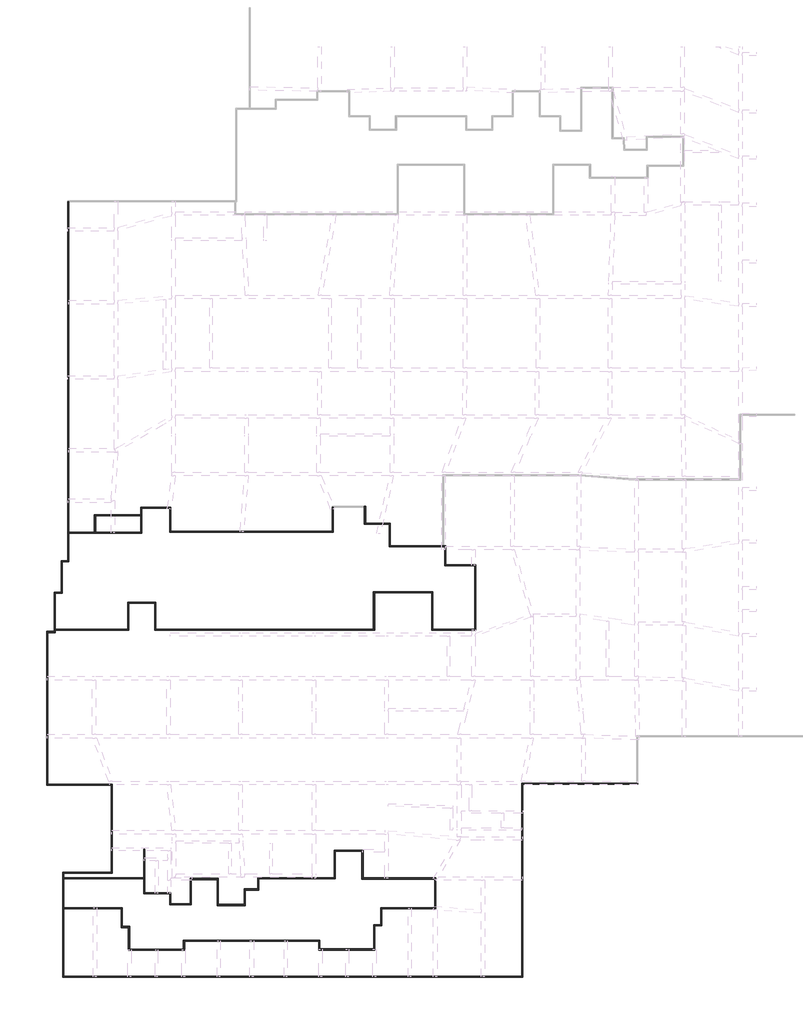
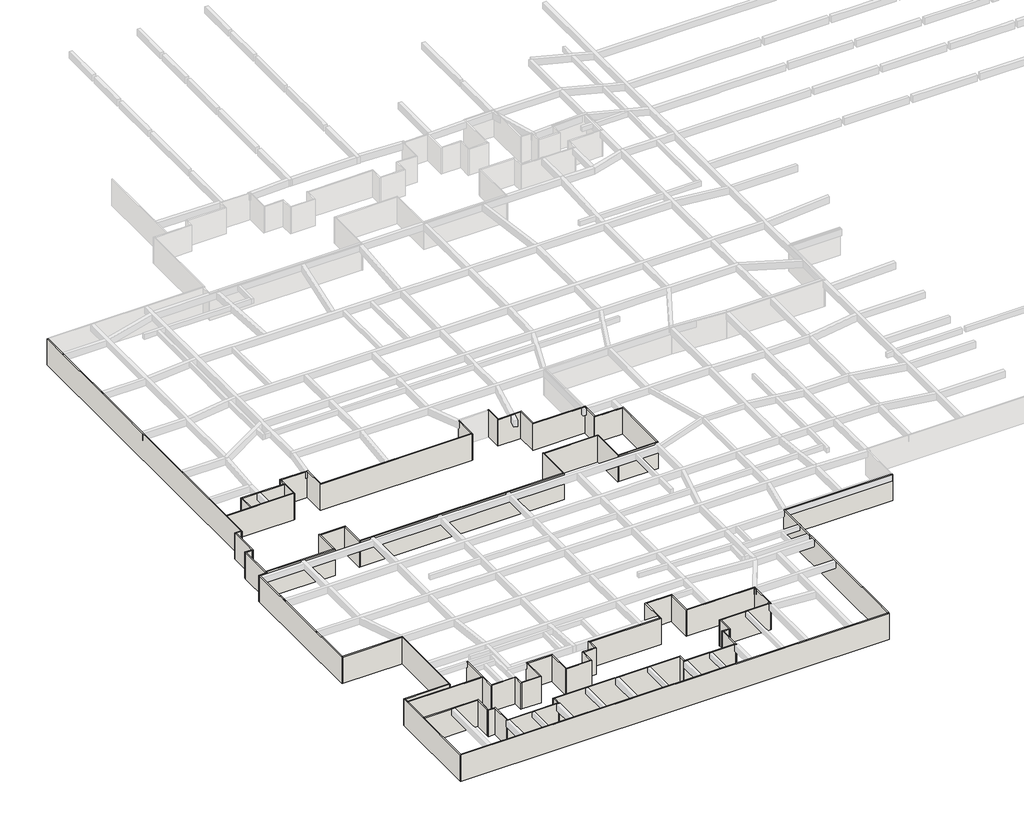
# One storey, part 1 of 16: 69 walls.
"""IFC4 building model written with IfcOpenShell, lengths in millimetres."""

from ifc_helpers import new_model, si_unit, origin, origin_with_axes, place, context, project, spatial, polyline, outline, extrude, faceted_brep, element, save

model = new_model("IFC4")

# Units and contexts
model_context = context("Model", 3, world=origin())
ifc_project = project(units=[si_unit("LENGTHUNIT", "METRE", prefix="MILLI")], contexts=[model_context])

# Site, building, storey
site = spatial("IfcSite", under=ifc_project)
building = spatial("IfcBuilding", under=site)
storey = spatial("IfcBuildingStorey", under=building, Name="户型图", Elevation=0.0)

# Walls
placement = place(None, origin())
element("IfcWall", 1, ObjectType="所有墙体", at=placement, inside=storey, context=model_context, shape_type="Brep", body=[
    faceted_brep([(66562.5546537, 146202.3185248, 0.0), (66562.5546537, 106222.3185248, 0.0), (66562.5546537, 106102.3185248, 0.0), (66562.5546537, 106102.3185248, 3300.0), (66562.5546537, 106222.3185248, 3300.0), (66562.5546537, 146202.3185248, 3300.0), (66682.5546537, 146202.3185248, 0.0), (66682.5546537, 146202.3185248, 3300.0), (66682.5546537, 109414.5259701, 3300.0), (66682.5546537, 109294.5259701, 3300.0), (66682.5546537, 106102.3185248, 3300.0), (66682.5546537, 106102.3185248, 0.0), (66682.5546537, 109294.5259701, 0.0), (66682.5546537, 109414.5259701, 0.0)], [[[0, 1, 2, 3, 4, 5]], [[6, 7, 8, 9, 10, 11, 12, 13]], [[2, 1, 0, 6, 13, 12, 11]], [[5, 4, 3, 10, 9, 8, 7]], [[0, 5, 7, 6]], [[3, 2, 11, 10]]]),
])
element("IfcWall", 2, ObjectType="所有墙体", at=placement, inside=storey, context=model_context, shape_type="Brep", body=[
    faceted_brep([(66562.5546537, 106222.3185248, 0.0), (65862.5546537, 106222.3185248, 0.0), (65862.5546537, 106222.3185248, 3300.0), (66562.5546537, 106222.3185248, 3300.0), (66562.5546537, 106102.3185248, 0.0), (66562.5546537, 106102.3185248, 3300.0), (65982.5546537, 106102.3185248, 3300.0), (65862.5546537, 106102.3185248, 3300.0), (65862.5546537, 106102.3185248, 0.0), (65982.5546537, 106102.3185248, 0.0)], [[[0, 1, 2, 3]], [[4, 5, 6, 7, 8, 9]], [[1, 0, 4, 9, 8]], [[3, 2, 7, 6, 5]], [[0, 3, 5, 4]], [[2, 1, 8, 7]]]),
])
element("IfcWall", 3, ObjectType="所有墙体", at=placement, inside=storey, context=model_context, shape_type="Brep", body=[
    faceted_brep([(65862.5546537, 106102.3185248, 0.0), (65862.5546537, 102722.3185248, 0.0), (65862.5546537, 102602.3185248, 0.0), (65862.5546537, 102602.3185248, 3300.0), (65862.5546537, 102722.3185248, 3300.0), (65862.5546537, 106102.3185248, 3300.0), (65982.5546537, 106102.3185248, 0.0), (65982.5546537, 106102.3185248, 3300.0), (65982.5546537, 102602.3185248, 3300.0), (65982.5546537, 102602.3185248, 0.0)], [[[0, 1, 2, 3, 4, 5]], [[6, 7, 8, 9]], [[2, 1, 0, 6, 9]], [[5, 4, 3, 8, 7]], [[0, 5, 7, 6]], [[3, 2, 9, 8]]]),
])
element("IfcWall", 4, ObjectType="所有墙体", at=placement, inside=storey, context=model_context, shape_type="Brep", body=[
    faceted_brep([(65862.5546537, 102722.3185248, 0.0), (65062.3671537, 102722.3185248, 0.0), (65062.3671537, 102722.3185248, 3300.0), (65862.5546537, 102722.3185248, 3300.0), (65862.5546537, 102602.3185248, 0.0), (65862.5546537, 102602.3185248, 3300.0), (65182.3671537, 102602.3185248, 3300.0), (65062.3671537, 102602.3185248, 3300.0), (65062.3671537, 102602.3185248, 0.0), (65182.3671537, 102602.3185248, 0.0)], [[[0, 1, 2, 3]], [[4, 5, 6, 7, 8, 9]], [[1, 0, 4, 9, 8]], [[3, 2, 7, 6, 5]], [[0, 3, 5, 4]], [[2, 1, 8, 7]]]),
])
element("IfcWall", 5, ObjectType="所有墙体", at=placement, inside=storey, context=model_context, shape_type="Brep", body=[
    faceted_brep([(65062.3671537, 102602.3185248, 0.0), (65062.3671537, 98364.6119076, 0.0), (65062.3671537, 98244.6119076, 0.0), (65062.3671537, 98244.6119076, 3300.0), (65062.3671537, 98364.6119076, 3300.0), (65062.3671537, 102602.3185248, 3300.0), (65182.3671537, 102602.3185248, 0.0), (65182.3671537, 102602.3185248, 3300.0), (65182.3671537, 98614.6119076, 3300.0), (65182.3671537, 98494.6119076, 3300.0), (65182.3671537, 98244.6119076, 3300.0), (65182.3671537, 98244.6119076, 0.0), (65182.3671537, 98494.6119076, 0.0), (65182.3671537, 98614.6119076, 0.0)], [[[0, 1, 2, 3, 4, 5]], [[6, 7, 8, 9, 10, 11, 12, 13]], [[2, 1, 0, 6, 13, 12, 11]], [[5, 4, 3, 10, 9, 8, 7]], [[0, 5, 7, 6]], [[3, 2, 11, 10]]]),
])
element("IfcWall", 6, ObjectType="所有墙体", at=placement, inside=storey, context=model_context, shape_type="Brep", body=[
    faceted_brep([(65062.3671537, 98364.6119076, 0.0), (64221.0654488, 98364.6119076, 0.0), (64221.0654488, 98364.6119076, 3300.0), (65062.3671537, 98364.6119076, 3300.0), (65062.3671537, 98244.6119076, 0.0), (65062.3671537, 98244.6119076, 3300.0), (64341.0654488, 98244.6119076, 3300.0), (64221.0654488, 98244.6119076, 3300.0), (64221.0654488, 98244.6119076, 0.0), (64341.0654488, 98244.6119076, 0.0)], [[[0, 1, 2, 3]], [[4, 5, 6, 7, 8, 9]], [[1, 0, 4, 9, 8]], [[3, 2, 7, 6, 5]], [[0, 3, 5, 4]], [[2, 1, 8, 7]]]),
])
element("IfcWall", 7, ObjectType="所有墙体", at=placement, inside=storey, context=model_context, shape_type="Brep", body=[
    faceted_brep([(64221.0654488, 98244.6119076, 0.0), (64221.0654488, 81244.6119076, 0.0), (64221.0654488, 81244.6119076, 3300.0), (64221.0654488, 98244.6119076, 3300.0), (64341.0654488, 98244.6119076, 0.0), (64341.0654488, 98244.6119076, 3300.0), (64341.0654488, 81364.6119076, 3300.0), (64341.0654488, 81244.6119076, 3300.0), (64341.0654488, 81244.6119076, 0.0), (64341.0654488, 81364.6119076, 0.0)], [[[0, 1, 2, 3]], [[4, 5, 6, 7, 8, 9]], [[1, 0, 4, 9, 8]], [[3, 2, 7, 6, 5]], [[0, 3, 5, 4]], [[2, 1, 8, 7]]]),
])
element("IfcWall", 8, ObjectType="所有墙体", at=placement, inside=storey, context=model_context, shape_type="Brep", body=[
    faceted_brep([(64341.0654488, 81244.6119076, 0.0), (71421.0654488, 81244.6119076, 0.0), (71541.0654488, 81244.6119076, 0.0), (71541.0654488, 81244.6119076, 3300.0), (71421.0654488, 81244.6119076, 3300.0), (64341.0654488, 81244.6119076, 3300.0), (64341.0654488, 81364.6119076, 0.0), (64341.0654488, 81364.6119076, 3300.0), (71541.0654488, 81364.6119076, 3300.0), (71541.0654488, 81364.6119076, 0.0)], [[[0, 1, 2, 3, 4, 5]], [[6, 7, 8, 9]], [[2, 1, 0, 6, 9]], [[5, 4, 3, 8, 7]], [[0, 5, 7, 6]], [[3, 2, 9, 8]]]),
])
element("IfcWall", 9, ObjectType="所有墙体", at=placement, inside=storey, context=model_context, shape_type="Brep", body=[
    faceted_brep([(71421.0654488, 81244.6119076, 0.0), (71421.0654488, 71564.6119076, 0.0), (71421.0654488, 71444.6119076, 0.0), (71421.0654488, 71444.6119076, 3300.0), (71421.0654488, 71564.6119076, 3300.0), (71421.0654488, 81244.6119076, 3300.0), (71541.0654488, 81244.6119076, 0.0), (71541.0654488, 81244.6119076, 3300.0), (71541.0654488, 71444.6119076, 3300.0), (71541.0654488, 71444.6119076, 0.0)], [[[0, 1, 2, 3, 4, 5]], [[6, 7, 8, 9]], [[2, 1, 0, 6, 9]], [[5, 4, 3, 8, 7]], [[0, 5, 7, 6]], [[3, 2, 9, 8]]]),
])
element("IfcWall", 10, ObjectType="所有墙体", at=placement, inside=storey, context=model_context, shape_type="Brep", body=[
    faceted_brep([(71421.0654488, 71564.6119076, 0.0), (66021.0654488, 71564.6119076, 0.0), (66021.0654488, 71564.6119076, 3300.0), (71421.0654488, 71564.6119076, 3300.0), (71421.0654488, 71444.6119076, 0.0), (71421.0654488, 71444.6119076, 3300.0), (66141.0654488, 71444.6119076, 3300.0), (66021.0654488, 71444.6119076, 3300.0), (66021.0654488, 71444.6119076, 0.0), (66141.0654488, 71444.6119076, 0.0)], [[[0, 1, 2, 3]], [[4, 5, 6, 7, 8, 9]], [[1, 0, 4, 9, 8]], [[3, 2, 7, 6, 5]], [[0, 3, 5, 4]], [[2, 1, 8, 7]]]),
])
element("IfcWall", 11, ObjectType="所有墙体", at=placement, inside=storey, context=model_context, shape_type="Brep", body=[
    faceted_brep([(66021.0654488, 71444.6119076, 0.0), (66021.0654488, 59844.6119076, 0.0), (66021.0654488, 59844.6119076, 3300.0), (66021.0654488, 71444.6119076, 3300.0), (66141.0654488, 71444.6119076, 0.0), (66141.0654488, 71444.6119076, 3300.0), (66141.0654488, 70967.5572201, 3300.0), (66141.0654488, 70847.5572201, 3300.0), (66141.0654488, 67617.5941469, 3300.0), (66141.0654488, 67497.5941469, 3300.0), (66141.0654488, 59964.6119076, 3300.0), (66141.0654488, 59844.6119076, 3300.0), (66141.0654488, 59844.6119076, 0.0), (66141.0654488, 59964.6119076, 0.0), (66141.0654488, 67497.5941469, 0.0), (66141.0654488, 67617.5941469, 0.0), (66141.0654488, 70847.5572201, 0.0), (66141.0654488, 70967.5572201, 0.0)], [[[0, 1, 2, 3]], [[4, 5, 6, 7, 8, 9, 10, 11, 12, 13, 14, 15, 16, 17]], [[1, 0, 4, 17, 16, 15, 14, 13, 12]], [[3, 2, 11, 10, 9, 8, 7, 6, 5]], [[0, 3, 5, 4]], [[2, 1, 12, 11]]]),
])
element("IfcWall", 12, ObjectType="所有墙体", at=placement, inside=storey, context=model_context, shape_type="Brep", body=[
    faceted_brep([(66141.0654488, 59844.6119076, 0.0), (117241.0654488, 59844.6119076, 0.0), (117241.0654488, 59844.6119076, 3300.0), (66141.0654488, 59844.6119076, 3300.0), (66141.0654488, 59964.6119076, 0.0), (66141.0654488, 59964.6119076, 3300.0), (117121.0654488, 59964.6119076, 3300.0), (117241.0654488, 59964.6119076, 3300.0), (117241.0654488, 59964.6119076, 0.0), (117121.0654488, 59964.6119076, 0.0)], [[[0, 1, 2, 3]], [[4, 5, 6, 7, 8, 9]], [[1, 0, 4, 9, 8]], [[3, 2, 7, 6, 5]], [[0, 3, 5, 4]], [[2, 1, 8, 7]]]),
])
element("IfcWall", 13, ObjectType="所有墙体", at=placement, inside=storey, context=model_context, shape_type="Brep", body=[
    faceted_brep([(117241.0654488, 59964.6119076, 0.0), (117241.0654488, 81344.6119076, 0.0), (117241.0654488, 81464.6119076, 0.0), (117241.0654488, 81464.6119076, 3300.0), (117241.0654488, 81344.6119076, 3300.0), (117241.0654488, 59964.6119076, 3300.0), (117121.0654488, 59964.6119076, 0.0), (117121.0654488, 59964.6119076, 3300.0), (117121.0654488, 81464.6119076, 3300.0), (117121.0654488, 81464.6119076, 0.0)], [[[0, 1, 2, 3, 4, 5]], [[6, 7, 8, 9]], [[2, 1, 0, 6, 9]], [[5, 4, 3, 8, 7]], [[0, 5, 7, 6]], [[3, 2, 9, 8]]]),
])
element("IfcWall", 14, ObjectType="所有墙体", at=placement, inside=storey, context=model_context, shape_type="Brep", body=[
    faceted_brep([(117241.0654488, 81344.6119076, 0.0), (130041.0654488, 81344.6119076, 0.0), (130041.0654488, 81344.6119076, 3300.0), (117241.0654488, 81344.6119076, 3300.0), (117241.0654488, 81464.6119076, 0.0), (117241.0654488, 81464.6119076, 3300.0), (129921.0654488, 81464.6119076, 3300.0), (130041.0654488, 81464.6119076, 3300.0), (130041.0654488, 81464.6119076, 0.0), (129921.0654488, 81464.6119076, 0.0)], [[[0, 1, 2, 3]], [[4, 5, 6, 7, 8, 9]], [[1, 0, 4, 9, 8]], [[3, 2, 7, 6, 5]], [[0, 3, 5, 4]], [[2, 1, 8, 7]]]),
])
element("IfcWall", 15, ObjectType="所有墙体", at=placement, inside=storey, context=model_context, shape_type="Brep", body=[
    faceted_brep([(65182.3671537, 98494.6119076, 0.0), (73382.3671537, 98494.6119076, 0.0), (73382.3671537, 98494.6119076, 3300.0), (65182.3671537, 98494.6119076, 3300.0), (65182.3671537, 98614.6119076, 0.0), (65182.3671537, 98614.6119076, 3300.0), (73262.3671537, 98614.6119076, 3300.0), (73382.3671537, 98614.6119076, 3300.0), (73382.3671537, 98614.6119076, 0.0), (73262.3671537, 98614.6119076, 0.0)], [[[0, 1, 2, 3]], [[4, 5, 6, 7, 8, 9]], [[1, 0, 4, 9, 8]], [[3, 2, 7, 6, 5]], [[0, 3, 5, 4]], [[2, 1, 8, 7]]]),
])
element("IfcWall", 16, ObjectType="所有墙体", at=placement, inside=storey, context=model_context, shape_type="Brep", body=[
    faceted_brep([(73382.3671537, 98614.6119076, 0.0), (73382.3671537, 101494.6119076, 0.0), (73382.3671537, 101614.6119076, 0.0), (73382.3671537, 101614.6119076, 3300.0), (73382.3671537, 101494.6119076, 3300.0), (73382.3671537, 98614.6119076, 3300.0), (73262.3671537, 98614.6119076, 0.0), (73262.3671537, 98614.6119076, 3300.0), (73262.3671537, 101614.6119076, 3300.0), (73262.3671537, 101614.6119076, 0.0)], [[[0, 1, 2, 3, 4, 5]], [[6, 7, 8, 9]], [[2, 1, 0, 6, 9]], [[5, 4, 3, 8, 7]], [[0, 5, 7, 6]], [[3, 2, 9, 8]]]),
])
element("IfcWall", 17, ObjectType="所有墙体", at=placement, inside=storey, context=model_context, shape_type="Brep", body=[
    faceted_brep([(73382.3671537, 101494.6119076, 0.0), (76262.3671537, 101494.6119076, 0.0), (76382.3671537, 101494.6119076, 0.0), (76382.3671537, 101494.6119076, 3300.0), (76262.3671537, 101494.6119076, 3300.0), (73382.3671537, 101494.6119076, 3300.0), (73382.3671537, 101614.6119076, 0.0), (73382.3671537, 101614.6119076, 3300.0), (76382.3671537, 101614.6119076, 3300.0), (76382.3671537, 101614.6119076, 0.0)], [[[0, 1, 2, 3, 4, 5]], [[6, 7, 8, 9]], [[2, 1, 0, 6, 9]], [[5, 4, 3, 8, 7]], [[0, 5, 7, 6]], [[3, 2, 9, 8]]]),
])
element("IfcWall", 18, ObjectType="所有墙体", at=placement, inside=storey, context=model_context, shape_type="Brep", body=[
    faceted_brep([(76262.3671537, 101494.6119076, 0.0), (76262.3671537, 98494.6092221, 0.0), (76262.3671537, 98494.6092221, 3300.0), (76262.3671537, 101494.6119076, 3300.0), (76382.3671537, 101494.6119076, 0.0), (76382.3671537, 101494.6119076, 3300.0), (76382.3671537, 98614.6092221, 3300.0), (76382.3671537, 98494.6092221, 3300.0), (76382.3671537, 98494.6092221, 0.0), (76382.3671537, 98614.6092221, 0.0)], [[[0, 1, 2, 3]], [[4, 5, 6, 7, 8, 9]], [[1, 0, 4, 9, 8]], [[3, 2, 7, 6, 5]], [[0, 3, 5, 4]], [[2, 1, 8, 7]]]),
])
element("IfcWall", 19, ObjectType="所有墙体", at=placement, inside=storey, context=model_context, shape_type="Brep", body=[
    faceted_brep([(76382.3671537, 98494.6092221, 0.0), (100732.3549466, 98494.6092221, 0.0), (100732.3549466, 98494.6092221, 3300.0), (76382.3671537, 98494.6092221, 3300.0), (76382.3671537, 98614.6092221, 0.0), (76382.3671537, 98614.6092221, 3300.0), (100612.3549466, 98614.6092221, 3300.0), (100732.3549466, 98614.6092221, 3300.0), (100732.3549466, 98614.6092221, 0.0), (100612.3549466, 98614.6092221, 0.0)], [[[0, 1, 2, 3]], [[4, 5, 6, 7, 8, 9]], [[1, 0, 4, 9, 8]], [[3, 2, 7, 6, 5]], [[0, 3, 5, 4]], [[2, 1, 8, 7]]]),
])
element("IfcWall", 20, ObjectType="所有墙体", at=placement, inside=storey, context=model_context, shape_type="Brep", body=[
    faceted_brep([(100732.3549466, 98614.6092221, 0.0), (100732.3549466, 102644.6089779, 0.0), (100732.3549466, 102764.6089779, 0.0), (100732.3549466, 102764.6089779, 3300.0), (100732.3549466, 102644.6089779, 3300.0), (100732.3549466, 98614.6092221, 3300.0), (100612.3549466, 98614.6092221, 0.0), (100612.3549466, 98614.6092221, 3300.0), (100612.3549466, 102764.6089779, 3300.0), (100612.3549466, 102764.6089779, 0.0)], [[[0, 1, 2, 3, 4, 5]], [[6, 7, 8, 9]], [[2, 1, 0, 6, 9]], [[5, 4, 3, 8, 7]], [[0, 5, 7, 6]], [[3, 2, 9, 8]]]),
])
element("IfcWall", 21, ObjectType="所有墙体", at=placement, inside=storey, context=model_context, shape_type="Brep", body=[
    faceted_brep([(100732.3549466, 102644.6089779, 0.0), (107112.3549466, 102644.6089779, 0.0), (107232.3549466, 102644.6089779, 0.0), (107232.3549466, 102644.6089779, 3300.0), (107112.3549466, 102644.6089779, 3300.0), (100732.3549466, 102644.6089779, 3300.0), (100732.3549466, 102764.6089779, 0.0), (100732.3549466, 102764.6089779, 3300.0), (107232.3549466, 102764.6089779, 3300.0), (107232.3549466, 102764.6089779, 0.0)], [[[0, 1, 2, 3, 4, 5]], [[6, 7, 8, 9]], [[2, 1, 0, 6, 9]], [[5, 4, 3, 8, 7]], [[0, 5, 7, 6]], [[3, 2, 9, 8]]]),
])
element("IfcWall", 22, ObjectType="所有墙体", at=placement, inside=storey, context=model_context, shape_type="Brep", body=[
    faceted_brep([(107112.3549466, 102644.6089779, 0.0), (107112.3549466, 98494.6092221, 0.0), (107112.3549466, 98494.6092221, 3300.0), (107112.3549466, 102644.6089779, 3300.0), (107232.3549466, 102644.6089779, 0.0), (107232.3549466, 102644.6089779, 3300.0), (107232.3549466, 98614.6092221, 3300.0), (107232.3549466, 98494.6092221, 3300.0), (107232.3549466, 98494.6092221, 0.0), (107232.3549466, 98614.6092221, 0.0)], [[[0, 1, 2, 3]], [[4, 5, 6, 7, 8, 9]], [[1, 0, 4, 9, 8]], [[3, 2, 7, 6, 5]], [[0, 3, 5, 4]], [[2, 1, 8, 7]]]),
])
element("IfcWall", 23, ObjectType="所有墙体", at=placement, inside=storey, context=model_context, shape_type="Brep", body=[
    faceted_brep([(107232.3549466, 98494.6092221, 0.0), (111982.3392399, 98494.6092221, 0.0), (111982.3392399, 98494.6092221, 3300.0), (107232.3549466, 98494.6092221, 3300.0), (107232.3549466, 98614.6092221, 0.0), (107232.3549466, 98614.6092221, 3300.0), (111862.3392399, 98614.6092221, 3300.0), (111982.3392399, 98614.6092221, 3300.0), (111982.3392399, 98614.6092221, 0.0), (111862.3392399, 98614.6092221, 0.0)], [[[0, 1, 2, 3]], [[4, 5, 6, 7, 8, 9]], [[1, 0, 4, 9, 8]], [[3, 2, 7, 6, 5]], [[0, 3, 5, 4]], [[2, 1, 8, 7]]]),
])
element("IfcWall", 24, ObjectType="所有墙体", at=placement, inside=storey, context=model_context, shape_type="Brep", body=[
    faceted_brep([(111982.3392399, 98614.6092221, 0.0), (111982.3392399, 105814.6092221, 0.0), (111982.3392399, 105814.6092221, 3300.0), (111982.3392399, 98614.6092221, 3300.0), (111862.3392399, 98614.6092221, 0.0), (111862.3392399, 98614.6092221, 3300.0), (111862.3392399, 105694.6092221, 3300.0), (111862.3392399, 105814.6092221, 3300.0), (111862.3392399, 105814.6092221, 0.0), (111862.3392399, 105694.6092221, 0.0)], [[[0, 1, 2, 3]], [[4, 5, 6, 7, 8, 9]], [[1, 0, 4, 9, 8]], [[3, 2, 7, 6, 5]], [[0, 3, 5, 4]], [[2, 1, 8, 7]]]),
])
element("IfcWall", 25, ObjectType="所有墙体", at=placement, inside=storey, context=model_context, shape_type="Brep", body=[
    faceted_brep([(111862.3392399, 105814.6092221, 0.0), (108682.3515287, 105814.6092221, 0.0), (108562.3515287, 105814.6092221, 0.0), (108562.3515287, 105814.6092221, 3300.0), (108682.3515287, 105814.6092221, 3300.0), (111862.3392399, 105814.6092221, 3300.0), (111862.3392399, 105694.6092221, 0.0), (111862.3392399, 105694.6092221, 3300.0), (108562.3515287, 105694.6092221, 3300.0), (108562.3515287, 105694.6092221, 0.0)], [[[0, 1, 2, 3, 4, 5]], [[6, 7, 8, 9]], [[2, 1, 0, 6, 9]], [[5, 4, 3, 8, 7]], [[0, 5, 7, 6]], [[3, 2, 9, 8]]]),
])
element("IfcWall", 26, ObjectType="所有墙体", at=placement, inside=storey, context=model_context, shape_type="Brep", body=[
    faceted_brep([(108682.3515287, 105814.6092221, 0.0), (108682.3515287, 107920.5715249, 0.0), (108682.3515287, 107920.5715249, 3300.0), (108682.3515287, 105814.6092221, 3300.0), (108562.3515287, 105814.6092221, 0.0), (108562.3515287, 105814.6092221, 3300.0), (108562.3515287, 107800.5715249, 3300.0), (108562.3515287, 107920.5715249, 3300.0), (108562.3515287, 107920.5715249, 0.0), (108562.3515287, 107800.5715249, 0.0)], [[[0, 1, 2, 3]], [[4, 5, 6, 7, 8, 9]], [[1, 0, 4, 9, 8]], [[3, 2, 7, 6, 5]], [[0, 3, 5, 4]], [[2, 1, 8, 7]]]),
])
element("IfcWall", 27, ObjectType="所有墙体", at=placement, inside=storey, context=model_context, shape_type="Brep", body=[
    faceted_brep([(108562.3515287, 107920.5715249, 0.0), (108444.4540331, 107920.5715249, 0.0), (108324.4540331, 107920.5715249, 0.0), (102482.3515287, 107920.5715249, 0.0), (102362.3515287, 107920.5715249, 0.0), (102362.3515287, 107920.5715249, 3300.0), (102482.3515287, 107920.5715249, 3300.0), (108324.4540331, 107920.5715249, 3300.0), (108444.4540331, 107920.5715249, 3300.0), (108562.3515287, 107920.5715249, 3300.0), (108562.3515287, 107800.5715249, 0.0), (108562.3515287, 107800.5715249, 3300.0), (102362.3515287, 107800.5715249, 3300.0), (102362.3515287, 107800.5715249, 0.0)], [[[0, 1, 2, 3, 4, 5, 6, 7, 8, 9]], [[10, 11, 12, 13]], [[4, 3, 2, 1, 0, 10, 13]], [[9, 8, 7, 6, 5, 12, 11]], [[0, 9, 11, 10]], [[5, 4, 13, 12]]]),
])
element("IfcWall", 28, ObjectType="所有墙体", at=placement, inside=storey, context=model_context, shape_type="Brep", body=[
    faceted_brep([(102482.3515287, 107920.5715249, 0.0), (102482.3515287, 110420.5715249, 0.0), (102482.3515287, 110420.5715249, 3300.0), (102482.3515287, 107920.5715249, 3300.0), (102362.3515287, 107920.5715249, 0.0), (102362.3515287, 107920.5715249, 3300.0), (102362.3515287, 110300.5715249, 3300.0), (102362.3515287, 110420.5715249, 3300.0), (102362.3515287, 110420.5715249, 0.0), (102362.3515287, 110300.5715249, 0.0)], [[[0, 1, 2, 3]], [[4, 5, 6, 7, 8, 9]], [[1, 0, 4, 9, 8]], [[3, 2, 7, 6, 5]], [[0, 3, 5, 4]], [[2, 1, 8, 7]]]),
])
element("IfcWall", 29, ObjectType="所有墙体", at=placement, inside=storey, context=model_context, shape_type="Brep", body=[
    faceted_brep([(102362.3515287, 110420.5715249, 0.0), (99732.3510404, 110420.5715249, 0.0), (99612.3510404, 110420.5715249, 0.0), (99612.3510404, 110420.5715249, 3300.0), (99732.3510404, 110420.5715249, 3300.0), (102362.3515287, 110420.5715249, 3300.0), (102362.3515287, 110300.5715249, 0.0), (102362.3515287, 110300.5715249, 3300.0), (99612.3510404, 110300.5715249, 3300.0), (99612.3510404, 110300.5715249, 0.0)], [[[0, 1, 2, 3, 4, 5]], [[6, 7, 8, 9]], [[2, 1, 0, 6, 9]], [[5, 4, 3, 8, 7]], [[0, 5, 7, 6]], [[3, 2, 9, 8]]]),
])
element("IfcWall", 30, ObjectType="所有墙体", at=placement, inside=storey, context=model_context, shape_type="Brep", body=[
    faceted_brep([(99732.3510404, 110420.5715249, 0.0), (99732.3510404, 112314.5259701, 0.0), (99732.3510404, 112314.5259701, 3300.0), (99732.3510404, 110420.5715249, 3300.0), (99612.3510404, 110420.5715249, 0.0), (99612.3510404, 110420.5715249, 3300.0), (99612.3510404, 112194.5259701, 3300.0), (99612.3510404, 112314.5259701, 3300.0), (99612.3510404, 112314.5259701, 0.0), (99612.3510404, 112194.5259701, 0.0)], [[[0, 1, 2, 3]], [[4, 5, 6, 7, 8, 9]], [[1, 0, 4, 9, 8]], [[3, 2, 7, 6, 5]], [[0, 3, 5, 4]], [[2, 1, 8, 7]]]),
])
element("IfcWall", 31, ObjectType="所有墙体", at=placement, inside=storey, context=model_context, shape_type="Brep", body=[
    faceted_brep([(96012.3510404, 112194.5259701, 0.0), (96012.3510404, 109514.5259701, 0.0), (96012.3510404, 109394.5259701, 0.0), (96012.3510404, 109394.5259701, 3300.0), (96012.3510404, 109514.5259701, 3300.0), (96012.3510404, 112194.5259701, 3300.0), (96132.3510404, 112194.5259701, 0.0), (96132.3510404, 112194.5259701, 3300.0), (96132.3510404, 109394.5259701, 3300.0), (96132.3510404, 109394.5259701, 0.0)], [[[0, 1, 2, 3, 4, 5]], [[6, 7, 8, 9]], [[2, 1, 0, 6, 9]], [[5, 4, 3, 8, 7]], [[0, 5, 7, 6]], [[3, 2, 9, 8]]]),
])
element("IfcWall", 32, ObjectType="所有墙体", at=placement, inside=storey, context=model_context, shape_type="Brep", body=[
    faceted_brep([(96012.3510404, 109514.5259701, 0.0), (78032.3510404, 109514.5259701, 0.0), (77912.3510404, 109514.5259701, 0.0), (77912.3510404, 109514.5259701, 3300.0), (78032.3510404, 109514.5259701, 3300.0), (96012.3510404, 109514.5259701, 3300.0), (96012.3510404, 109394.5259701, 0.0), (96012.3510404, 109394.5259701, 3300.0), (77912.3510404, 109394.5259701, 3300.0), (77912.3510404, 109394.5259701, 0.0)], [[[0, 1, 2, 3, 4, 5]], [[6, 7, 8, 9]], [[2, 1, 0, 6, 9]], [[5, 4, 3, 8, 7]], [[0, 5, 7, 6]], [[3, 2, 9, 8]]]),
])
element("IfcWall", 33, ObjectType="所有墙体", at=placement, inside=storey, context=model_context, shape_type="Brep", body=[
    faceted_brep([(78032.3510404, 109514.5259701, 0.0), (78032.3510404, 112214.5259701, 0.0), (78032.3510404, 112214.5259701, 3300.0), (78032.3510404, 109514.5259701, 3300.0), (77912.3510404, 109514.5259701, 0.0), (77912.3510404, 109514.5259701, 3300.0), (77912.3510404, 112094.5259701, 3300.0), (77912.3510404, 112214.5259701, 3300.0), (77912.3510404, 112214.5259701, 0.0), (77912.3510404, 112094.5259701, 0.0)], [[[0, 1, 2, 3]], [[4, 5, 6, 7, 8, 9]], [[1, 0, 4, 9, 8]], [[3, 2, 7, 6, 5]], [[0, 3, 5, 4]], [[2, 1, 8, 7]]]),
])
element("IfcWall", 34, ObjectType="所有墙体", at=placement, inside=storey, context=model_context, shape_type="Brep", body=[
    faceted_brep([(77912.3510404, 112214.5259701, 0.0), (74712.3510404, 112214.5259701, 0.0), (74712.3510404, 112214.5259701, 3300.0), (77912.3510404, 112214.5259701, 3300.0), (77912.3510404, 112094.5259701, 0.0), (77912.3510404, 112094.5259701, 3300.0), (74832.3510404, 112094.5259701, 3300.0), (74712.3510404, 112094.5259701, 3300.0), (74712.3510404, 112094.5259701, 0.0), (74832.3510404, 112094.5259701, 0.0)], [[[0, 1, 2, 3]], [[4, 5, 6, 7, 8, 9]], [[1, 0, 4, 9, 8]], [[3, 2, 7, 6, 5]], [[0, 3, 5, 4]], [[2, 1, 8, 7]]]),
])
element("IfcWall", 35, ObjectType="所有墙体", at=placement, inside=storey, context=model_context, shape_type="Brep", body=[
    faceted_brep([(74712.3510404, 112094.5259701, 0.0), (74712.3510404, 111354.5259701, 0.0), (74712.3510404, 111234.5259701, 0.0), (74712.3510404, 109414.5259701, 0.0), (74712.3510404, 109294.5259701, 0.0), (74712.3510404, 109294.5259701, 3300.0), (74712.3510404, 109414.5259701, 3300.0), (74712.3510404, 111234.5259701, 3300.0), (74712.3510404, 111354.5259701, 3300.0), (74712.3510404, 112094.5259701, 3300.0), (74832.3510404, 112094.5259701, 0.0), (74832.3510404, 112094.5259701, 3300.0), (74832.3510404, 109294.5259701, 3300.0), (74832.3510404, 109294.5259701, 0.0)], [[[0, 1, 2, 3, 4, 5, 6, 7, 8, 9]], [[10, 11, 12, 13]], [[4, 3, 2, 1, 0, 10, 13]], [[9, 8, 7, 6, 5, 12, 11]], [[0, 9, 11, 10]], [[5, 4, 13, 12]]]),
])
element("IfcWall", 36, ObjectType="所有墙体", at=placement, inside=storey, context=model_context, shape_type="Brep", body=[
    faceted_brep([(74712.3510404, 109414.5259701, 0.0), (69672.3510404, 109414.5259701, 0.0), (69552.3510404, 109414.5259701, 0.0), (66682.5546537, 109414.5259701, 0.0), (66682.5546537, 109414.5259701, 3300.0), (69552.3510404, 109414.5259701, 3300.0), (69672.3510404, 109414.5259701, 3300.0), (74712.3510404, 109414.5259701, 3300.0), (74712.3510404, 109294.5259701, 0.0), (74712.3510404, 109294.5259701, 3300.0), (66682.5546537, 109294.5259701, 3300.0), (66682.5546537, 109294.5259701, 0.0)], [[[0, 1, 2, 3, 4, 5, 6, 7]], [[8, 9, 10, 11]], [[3, 2, 1, 0, 8, 11]], [[7, 6, 5, 4, 10, 9]], [[0, 7, 9, 8]], [[4, 3, 11, 10]]]),
])
element("IfcWall", 37, ObjectType="所有墙体", at=placement, inside=storey, context=model_context, shape_type="Brep", body=[
    faceted_brep([(74712.3510404, 111354.5259701, 0.0), (69552.3510404, 111354.5259701, 0.0), (69552.3510404, 111354.5259701, 3300.0), (74712.3510404, 111354.5259701, 3300.0), (74712.3510404, 111234.5259701, 0.0), (74712.3510404, 111234.5259701, 3300.0), (69672.3510404, 111234.5259701, 3300.0), (69552.3510404, 111234.5259701, 3300.0), (69552.3510404, 111234.5259701, 0.0), (69672.3510404, 111234.5259701, 0.0)], [[[0, 1, 2, 3]], [[4, 5, 6, 7, 8, 9]], [[1, 0, 4, 9, 8]], [[3, 2, 7, 6, 5]], [[0, 3, 5, 4]], [[2, 1, 8, 7]]]),
])
element("IfcWall", 38, ObjectType="所有墙体", at=placement, inside=storey, context=model_context, shape_type="SweptSolid", body=[
    extrude(outline(polyline([(69552.3510404, 109414.5259701), (69552.3510404, 111234.5259701), (69672.3510404, 111234.5259701), (69672.3510404, 109414.5259701), (69552.3510404, 109414.5259701)])), origin_with_axes(), (0.0, 0.0, 1.0), 3300.0),
])
element("IfcWall", 39, ObjectType="所有墙体", at=placement, inside=storey, context=model_context, shape_type="SweptSolid", body=[
    extrude(outline(polyline([(75021.0654488, 70847.5572201), (66141.0654488, 70847.5572201), (66141.0654488, 70967.5572201), (75021.0654488, 70967.5572201), (75021.0654488, 70847.5572201)])), origin_with_axes(), (0.0, 0.0, 1.0), 3300.0),
])
element("IfcWall", 40, ObjectType="所有墙体", at=placement, inside=storey, context=model_context, shape_type="Brep", body=[
    faceted_brep([(75141.0654488, 69147.5572201, 0.0), (75141.0654488, 69267.5572201, 0.0), (75141.0654488, 74107.5572201, 0.0), (75141.0654488, 74107.5572201, 3300.0), (75141.0654488, 69267.5572201, 3300.0), (75141.0654488, 69147.5572201, 3300.0), (75021.0654488, 69147.5572201, 0.0), (75021.0654488, 69147.5572201, 3300.0), (75021.0654488, 70847.5572201, 3300.0), (75021.0654488, 70967.5572201, 3300.0), (75021.0654488, 74107.5572201, 3300.0), (75021.0654488, 74107.5572201, 0.0), (75021.0654488, 70967.5572201, 0.0), (75021.0654488, 70847.5572201, 0.0)], [[[0, 1, 2, 3, 4, 5]], [[6, 7, 8, 9, 10, 11, 12, 13]], [[2, 1, 0, 6, 13, 12, 11]], [[3, 2, 11, 10]], [[5, 4, 3, 10, 9, 8, 7]], [[0, 5, 7, 6]]]),
])
element("IfcWall", 41, ObjectType="所有墙体", at=placement, inside=storey, context=model_context, shape_type="Brep", body=[
    faceted_brep([(75141.0654488, 69147.5572201, 0.0), (77937.2421537, 69147.5572201, 0.0), (78057.2421537, 69147.5572201, 0.0), (78057.2421537, 69147.5572201, 3300.0), (77937.2421537, 69147.5572201, 3300.0), (75141.0654488, 69147.5572201, 3300.0), (75141.0654488, 69267.5572201, 0.0), (75141.0654488, 69267.5572201, 3300.0), (78057.2421537, 69267.5572201, 3300.0), (78057.2421537, 69267.5572201, 0.0)], [[[0, 1, 2, 3, 4, 5]], [[6, 7, 8, 9]], [[2, 1, 0, 6, 9]], [[5, 4, 3, 8, 7]], [[0, 5, 7, 6]], [[3, 2, 9, 8]]]),
])
element("IfcWall", 42, ObjectType="所有墙体", at=placement, inside=storey, context=model_context, shape_type="Brep", body=[
    faceted_brep([(77937.2421537, 69147.5572201, 0.0), (77937.2421537, 67947.5572201, 0.0), (77937.2421537, 67947.5572201, 3300.0), (77937.2421537, 69147.5572201, 3300.0), (78057.2421537, 69147.5572201, 0.0), (78057.2421537, 69147.5572201, 3300.0), (78057.2421537, 68067.5572201, 3300.0), (78057.2421537, 67947.5572201, 3300.0), (78057.2421537, 67947.5572201, 0.0), (78057.2421537, 68067.5572201, 0.0)], [[[0, 1, 2, 3]], [[4, 5, 6, 7, 8, 9]], [[1, 0, 4, 9, 8]], [[3, 2, 7, 6, 5]], [[0, 3, 5, 4]], [[2, 1, 8, 7]]]),
])
element("IfcWall", 43, ObjectType="所有墙体", at=placement, inside=storey, context=model_context, shape_type="Brep", body=[
    faceted_brep([(78057.2421537, 67947.5572201, 0.0), (80357.2421537, 67947.5572201, 0.0), (80357.2421537, 67947.5572201, 3300.0), (78057.2421537, 67947.5572201, 3300.0), (78057.2421537, 68067.5572201, 0.0), (78057.2421537, 68067.5572201, 3300.0), (80237.2421537, 68067.5572201, 3300.0), (80357.2421537, 68067.5572201, 3300.0), (80357.2421537, 68067.5572201, 0.0), (80237.2421537, 68067.5572201, 0.0)], [[[0, 1, 2, 3]], [[4, 5, 6, 7, 8, 9]], [[1, 0, 4, 9, 8]], [[3, 2, 7, 6, 5]], [[0, 3, 5, 4]], [[2, 1, 8, 7]]]),
])
element("IfcWall", 44, ObjectType="所有墙体", at=placement, inside=storey, context=model_context, shape_type="Brep", body=[
    faceted_brep([(80357.2421537, 68067.5572201, 0.0), (80357.2421537, 70747.5572201, 0.0), (80357.2421537, 70867.5572201, 0.0), (80357.2421537, 70867.5572201, 3300.0), (80357.2421537, 70747.5572201, 3300.0), (80357.2421537, 68067.5572201, 3300.0), (80237.2421537, 68067.5572201, 0.0), (80237.2421537, 68067.5572201, 3300.0), (80237.2421537, 70867.5572201, 3300.0), (80237.2421537, 70867.5572201, 0.0)], [[[0, 1, 2, 3, 4, 5]], [[6, 7, 8, 9]], [[2, 1, 0, 6, 9]], [[5, 4, 3, 8, 7]], [[0, 5, 7, 6]], [[3, 2, 9, 8]]]),
])
element("IfcWall", 45, ObjectType="所有墙体", at=placement, inside=storey, context=model_context, shape_type="Brep", body=[
    faceted_brep([(80357.2421537, 70747.5572201, 0.0), (83237.2421537, 70747.5572201, 0.0), (83357.2421537, 70747.5572201, 0.0), (83357.2421537, 70747.5572201, 3300.0), (83237.2421537, 70747.5572201, 3300.0), (80357.2421537, 70747.5572201, 3300.0), (80357.2421537, 70867.5572201, 0.0), (80357.2421537, 70867.5572201, 3300.0), (83357.2421537, 70867.5572201, 3300.0), (83357.2421537, 70867.5572201, 0.0)], [[[0, 1, 2, 3, 4, 5]], [[6, 7, 8, 9]], [[2, 1, 0, 6, 9]], [[5, 4, 3, 8, 7]], [[0, 5, 7, 6]], [[3, 2, 9, 8]]]),
])
element("IfcWall", 46, ObjectType="所有墙体", at=placement, inside=storey, context=model_context, shape_type="Brep", body=[
    faceted_brep([(83237.2421537, 70747.5572201, 0.0), (83237.2421537, 67847.5572201, 0.0), (83237.2421537, 67847.5572201, 3300.0), (83237.2421537, 70747.5572201, 3300.0), (83357.2421537, 70747.5572201, 0.0), (83357.2421537, 70747.5572201, 3300.0), (83357.2421537, 67967.5572201, 3300.0), (83357.2421537, 67847.5572201, 3300.0), (83357.2421537, 67847.5572201, 0.0), (83357.2421537, 67967.5572201, 0.0)], [[[0, 1, 2, 3]], [[4, 5, 6, 7, 8, 9]], [[1, 0, 4, 9, 8]], [[3, 2, 7, 6, 5]], [[0, 3, 5, 4]], [[2, 1, 8, 7]]]),
])
element("IfcWall", 47, ObjectType="所有墙体", at=placement, inside=storey, context=model_context, shape_type="Brep", body=[
    faceted_brep([(83357.2421537, 67847.5572201, 0.0), (86357.2421537, 67847.5572201, 0.0), (86357.2421537, 67847.5572201, 3300.0), (83357.2421537, 67847.5572201, 3300.0), (83357.2421537, 67967.5572201, 0.0), (83357.2421537, 67967.5572201, 3300.0), (86237.2421537, 67967.5572201, 3300.0), (86357.2421537, 67967.5572201, 3300.0), (86357.2421537, 67967.5572201, 0.0), (86237.2421537, 67967.5572201, 0.0)], [[[0, 1, 2, 3]], [[4, 5, 6, 7, 8, 9]], [[1, 0, 4, 9, 8]], [[3, 2, 7, 6, 5]], [[0, 3, 5, 4]], [[2, 1, 8, 7]]]),
])
element("IfcWall", 48, ObjectType="所有墙体", at=placement, inside=storey, context=model_context, shape_type="Brep", body=[
    faceted_brep([(86357.2421537, 67967.5572201, 0.0), (86357.2421537, 69572.5572201, 0.0), (86357.2421537, 69692.5572201, 0.0), (86357.2421537, 69692.5572201, 3300.0), (86357.2421537, 69572.5572201, 3300.0), (86357.2421537, 67967.5572201, 3300.0), (86237.2421537, 67967.5572201, 0.0), (86237.2421537, 67967.5572201, 3300.0), (86237.2421537, 69692.5572201, 3300.0), (86237.2421537, 69692.5572201, 0.0)], [[[0, 1, 2, 3, 4, 5]], [[6, 7, 8, 9]], [[2, 1, 0, 6, 9]], [[5, 4, 3, 8, 7]], [[0, 5, 7, 6]], [[3, 2, 9, 8]]]),
])
element("IfcWall", 49, ObjectType="所有墙体", at=placement, inside=storey, context=model_context, shape_type="Brep", body=[
    faceted_brep([(86357.2421537, 69572.5572201, 0.0), (87857.242764, 69572.5572201, 0.0), (87857.242764, 69572.5572201, 3300.0), (86357.2421537, 69572.5572201, 3300.0), (86357.2421537, 69692.5572201, 0.0), (86357.2421537, 69692.5572201, 3300.0), (87737.242764, 69692.5572201, 3300.0), (87857.242764, 69692.5572201, 3300.0), (87857.242764, 69692.5572201, 0.0), (87737.242764, 69692.5572201, 0.0)], [[[0, 1, 2, 3]], [[4, 5, 6, 7, 8, 9]], [[1, 0, 4, 9, 8]], [[3, 2, 7, 6, 5]], [[0, 3, 5, 4]], [[2, 1, 8, 7]]]),
])
element("IfcWall", 50, ObjectType="所有墙体", at=placement, inside=storey, context=model_context, shape_type="Brep", body=[
    faceted_brep([(87857.242764, 69692.5572201, 0.0), (87857.242764, 70847.5521192, 0.0), (87857.242764, 70967.5521192, 0.0), (87857.242764, 70967.5521192, 3300.0), (87857.242764, 70847.5521192, 3300.0), (87857.242764, 69692.5572201, 3300.0), (87737.242764, 69692.5572201, 0.0), (87737.242764, 69692.5572201, 3300.0), (87737.242764, 70967.5521192, 3300.0), (87737.242764, 70967.5521192, 0.0)], [[[0, 1, 2, 3, 4, 5]], [[6, 7, 8, 9]], [[2, 1, 0, 6, 9]], [[5, 4, 3, 8, 7]], [[0, 5, 7, 6]], [[3, 2, 9, 8]]]),
])
element("IfcWall", 51, ObjectType="所有墙体", at=placement, inside=storey, context=model_context, shape_type="Brep", body=[
    faceted_brep([(87857.242764, 70847.5521192, 0.0), (96357.242764, 70847.5521192, 0.0), (96357.242764, 70847.5521192, 3300.0), (87857.242764, 70847.5521192, 3300.0), (87857.242764, 70967.5521192, 0.0), (87857.242764, 70967.5521192, 3300.0), (96237.242764, 70967.5521192, 3300.0), (96357.242764, 70967.5521192, 3300.0), (96357.242764, 70967.5521192, 0.0), (96237.242764, 70967.5521192, 0.0)], [[[0, 1, 2, 3]], [[4, 5, 6, 7, 8, 9]], [[1, 0, 4, 9, 8]], [[3, 2, 7, 6, 5]], [[0, 3, 5, 4]], [[2, 1, 8, 7]]]),
])
element("IfcWall", 52, ObjectType="所有墙体", at=placement, inside=storey, context=model_context, shape_type="Brep", body=[
    faceted_brep([(96357.242764, 70967.5521192, 0.0), (96357.242764, 73897.5941469, 0.0), (96357.242764, 74017.5941469, 0.0), (96357.242764, 74017.5941469, 3300.0), (96357.242764, 73897.5941469, 3300.0), (96357.242764, 70967.5521192, 3300.0), (96237.242764, 70967.5521192, 0.0), (96237.242764, 70967.5521192, 3300.0), (96237.242764, 74017.5941469, 3300.0), (96237.242764, 74017.5941469, 0.0)], [[[0, 1, 2, 3, 4, 5]], [[6, 7, 8, 9]], [[2, 1, 0, 6, 9]], [[5, 4, 3, 8, 7]], [[0, 5, 7, 6]], [[3, 2, 9, 8]]]),
])
element("IfcWall", 53, ObjectType="所有墙体", at=placement, inside=storey, context=model_context, shape_type="Brep", body=[
    faceted_brep([(96357.242764, 73897.5941469, 0.0), (99335.5415162, 73897.5941469, 0.0), (99455.5415162, 73897.5941469, 0.0), (99455.5415162, 73897.5941469, 3300.0), (99335.5415162, 73897.5941469, 3300.0), (96357.242764, 73897.5941469, 3300.0), (96357.242764, 74017.5941469, 0.0), (96357.242764, 74017.5941469, 3300.0), (99455.5415162, 74017.5941469, 3300.0), (99455.5415162, 74017.5941469, 0.0)], [[[0, 1, 2, 3, 4, 5]], [[6, 7, 8, 9]], [[2, 1, 0, 6, 9]], [[5, 4, 3, 8, 7]], [[0, 5, 7, 6]], [[3, 2, 9, 8]]]),
])
element("IfcWall", 54, ObjectType="所有墙体", at=placement, inside=storey, context=model_context, shape_type="Brep", body=[
    faceted_brep([(99335.5415162, 73897.5941469, 0.0), (99335.5415162, 70797.5941469, 0.0), (99335.5415162, 70797.5941469, 3300.0), (99335.5415162, 73897.5941469, 3300.0), (99455.5415162, 73897.5941469, 0.0), (99455.5415162, 73897.5941469, 3300.0), (99455.5415162, 70917.5941469, 3300.0), (99455.5415162, 70797.5941469, 3300.0), (99455.5415162, 70797.5941469, 0.0), (99455.5415162, 70917.5941469, 0.0)], [[[0, 1, 2, 3]], [[4, 5, 6, 7, 8, 9]], [[1, 0, 4, 9, 8]], [[3, 2, 7, 6, 5]], [[0, 3, 5, 4]], [[2, 1, 8, 7]]]),
])
element("IfcWall", 55, ObjectType="所有墙体", at=placement, inside=storey, context=model_context, shape_type="Brep", body=[
    faceted_brep([(99455.5415162, 70797.5941469, 0.0), (107435.5415162, 70797.5941469, 0.0), (107555.5415162, 70797.5941469, 0.0), (107555.5415162, 70797.5941469, 3300.0), (107435.5415162, 70797.5941469, 3300.0), (99455.5415162, 70797.5941469, 3300.0), (99455.5415162, 70917.5941469, 0.0), (99455.5415162, 70917.5941469, 3300.0), (107555.5415162, 70917.5941469, 3300.0), (107555.5415162, 70917.5941469, 0.0)], [[[0, 1, 2, 3, 4, 5]], [[6, 7, 8, 9]], [[2, 1, 0, 6, 9]], [[5, 4, 3, 8, 7]], [[0, 5, 7, 6]], [[3, 2, 9, 8]]]),
])
element("IfcWall", 56, ObjectType="所有墙体", at=placement, inside=storey, context=model_context, shape_type="Brep", body=[
    faceted_brep([(107435.5415162, 70797.5941469, 0.0), (107435.5415162, 67617.5941469, 0.0), (107435.5415162, 67497.5941469, 0.0), (107435.5415162, 67497.5941469, 3300.0), (107435.5415162, 67617.5941469, 3300.0), (107435.5415162, 70797.5941469, 3300.0), (107555.5415162, 70797.5941469, 0.0), (107555.5415162, 70797.5941469, 3300.0), (107555.5415162, 67497.5941469, 3300.0), (107555.5415162, 67497.5941469, 0.0)], [[[0, 1, 2, 3, 4, 5]], [[6, 7, 8, 9]], [[2, 1, 0, 6, 9]], [[5, 4, 3, 8, 7]], [[0, 5, 7, 6]], [[3, 2, 9, 8]]]),
])
element("IfcWall", 57, ObjectType="所有墙体", at=placement, inside=storey, context=model_context, shape_type="Brep", body=[
    faceted_brep([(107435.5415162, 67617.5941469, 0.0), (101437.0218171, 67617.5941469, 0.0), (101437.0218171, 67617.5941469, 3300.0), (107435.5415162, 67617.5941469, 3300.0), (107435.5415162, 67497.5941469, 0.0), (107435.5415162, 67497.5941469, 3300.0), (101557.0218171, 67497.5941469, 3300.0), (101437.0218171, 67497.5941469, 3300.0), (101437.0218171, 67497.5941469, 0.0), (101557.0218171, 67497.5941469, 0.0)], [[[0, 1, 2, 3]], [[4, 5, 6, 7, 8, 9]], [[1, 0, 4, 9, 8]], [[3, 2, 7, 6, 5]], [[0, 3, 5, 4]], [[2, 1, 8, 7]]]),
])
element("IfcWall", 58, ObjectType="所有墙体", at=placement, inside=storey, context=model_context, shape_type="Brep", body=[
    faceted_brep([(101437.0218171, 67497.5941469, 0.0), (101437.0218171, 65717.5941469, 0.0), (101437.0218171, 65597.5941469, 0.0), (101437.0218171, 65597.5941469, 3300.0), (101437.0218171, 65717.5941469, 3300.0), (101437.0218171, 67497.5941469, 3300.0), (101557.0218171, 67497.5941469, 0.0), (101557.0218171, 67497.5941469, 3300.0), (101557.0218171, 65597.5941469, 3300.0), (101557.0218171, 65597.5941469, 0.0)], [[[0, 1, 2, 3, 4, 5]], [[6, 7, 8, 9]], [[2, 1, 0, 6, 9]], [[5, 4, 3, 8, 7]], [[0, 5, 7, 6]], [[3, 2, 9, 8]]]),
])
element("IfcWall", 59, ObjectType="所有墙体", at=placement, inside=storey, context=model_context, shape_type="Brep", body=[
    faceted_brep([(101437.0218171, 65717.5941469, 0.0), (100637.235631, 65717.5941469, 0.0), (100637.235631, 65717.5941469, 3300.0), (101437.0218171, 65717.5941469, 3300.0), (101437.0218171, 65597.5941469, 0.0), (101437.0218171, 65597.5941469, 3300.0), (100757.235631, 65597.5941469, 3300.0), (100637.235631, 65597.5941469, 3300.0), (100637.235631, 65597.5941469, 0.0), (100757.235631, 65597.5941469, 0.0)], [[[0, 1, 2, 3]], [[4, 5, 6, 7, 8, 9]], [[1, 0, 4, 9, 8]], [[3, 2, 7, 6, 5]], [[0, 3, 5, 4]], [[2, 1, 8, 7]]]),
])
element("IfcWall", 60, ObjectType="所有墙体", at=placement, inside=storey, context=model_context, shape_type="Brep", body=[
    faceted_brep([(100637.235631, 65597.5941469, 0.0), (100637.235631, 63017.5941469, 0.0), (100637.235631, 62897.5941469, 0.0), (100637.235631, 62897.5941469, 3300.0), (100637.235631, 63017.5941469, 3300.0), (100637.235631, 65597.5941469, 3300.0), (100757.235631, 65597.5941469, 0.0), (100757.235631, 65597.5941469, 3300.0), (100757.235631, 62897.5941469, 3300.0), (100757.235631, 62897.5941469, 0.0)], [[[0, 1, 2, 3, 4, 5]], [[6, 7, 8, 9]], [[2, 1, 0, 6, 9]], [[5, 4, 3, 8, 7]], [[0, 5, 7, 6]], [[3, 2, 9, 8]]]),
])
element("IfcWall", 61, ObjectType="所有墙体", at=placement, inside=storey, context=model_context, shape_type="Brep", body=[
    faceted_brep([(100637.235631, 63017.5941469, 0.0), (94657.2447171, 63017.5941469, 0.0), (94537.2447171, 63017.5941469, 0.0), (94537.2447171, 63017.5941469, 3300.0), (94657.2447171, 63017.5941469, 3300.0), (100637.235631, 63017.5941469, 3300.0), (100637.235631, 62897.5941469, 0.0), (100637.235631, 62897.5941469, 3300.0), (94537.2447171, 62897.5941469, 3300.0), (94537.2447171, 62897.5941469, 0.0)], [[[0, 1, 2, 3, 4, 5]], [[6, 7, 8, 9]], [[2, 1, 0, 6, 9]], [[5, 4, 3, 8, 7]], [[0, 5, 7, 6]], [[3, 2, 9, 8]]]),
])
element("IfcWall", 62, ObjectType="所有墙体", at=placement, inside=storey, context=model_context, shape_type="Brep", body=[
    faceted_brep([(94657.2447171, 63017.5941469, 0.0), (94657.2447171, 63967.635127, 0.0), (94657.2447171, 63967.635127, 3300.0), (94657.2447171, 63017.5941469, 3300.0), (94537.2447171, 63017.5941469, 0.0), (94537.2447171, 63017.5941469, 3300.0), (94537.2447171, 63847.635127, 3300.0), (94537.2447171, 63967.635127, 3300.0), (94537.2447171, 63967.635127, 0.0), (94537.2447171, 63847.635127, 0.0)], [[[0, 1, 2, 3]], [[4, 5, 6, 7, 8, 9]], [[1, 0, 4, 9, 8]], [[3, 2, 7, 6, 5]], [[0, 3, 5, 4]], [[2, 1, 8, 7]]]),
])
element("IfcWall", 63, ObjectType="所有墙体", at=placement, inside=storey, context=model_context, shape_type="Brep", body=[
    faceted_brep([(94537.2447171, 63967.635127, 0.0), (79462.242764, 63967.635127, 0.0), (79462.242764, 63967.635127, 3300.0), (94537.2447171, 63967.635127, 3300.0), (94537.2447171, 63847.635127, 0.0), (94537.2447171, 63847.635127, 3300.0), (79582.242764, 63847.635127, 3300.0), (79462.242764, 63847.635127, 3300.0), (79462.242764, 63847.635127, 0.0), (79582.242764, 63847.635127, 0.0)], [[[0, 1, 2, 3]], [[4, 5, 6, 7, 8, 9]], [[1, 0, 4, 9, 8]], [[3, 2, 7, 6, 5]], [[0, 3, 5, 4]], [[2, 1, 8, 7]]]),
])
element("IfcWall", 64, ObjectType="所有墙体", at=placement, inside=storey, context=model_context, shape_type="Brep", body=[
    faceted_brep([(79462.242764, 63847.635127, 0.0), (79462.242764, 62967.635127, 0.0), (79462.242764, 62847.635127, 0.0), (79462.242764, 62847.635127, 3300.0), (79462.242764, 62967.635127, 3300.0), (79462.242764, 63847.635127, 3300.0), (79582.242764, 63847.635127, 0.0), (79582.242764, 63847.635127, 3300.0), (79582.242764, 62847.635127, 3300.0), (79582.242764, 62847.635127, 0.0)], [[[0, 1, 2, 3, 4, 5]], [[6, 7, 8, 9]], [[2, 1, 0, 6, 9]], [[5, 4, 3, 8, 7]], [[0, 5, 7, 6]], [[3, 2, 9, 8]]]),
])
element("IfcWall", 65, ObjectType="所有墙体", at=placement, inside=storey, context=model_context, shape_type="Brep", body=[
    faceted_brep([(79462.242764, 62967.635127, 0.0), (73457.2408109, 62967.635127, 0.0), (73337.2408109, 62967.635127, 0.0), (73337.2408109, 62967.635127, 3300.0), (73457.2408109, 62967.635127, 3300.0), (79462.242764, 62967.635127, 3300.0), (79462.242764, 62847.635127, 0.0), (79462.242764, 62847.635127, 3300.0), (73337.2408109, 62847.635127, 3300.0), (73337.2408109, 62847.635127, 0.0)], [[[0, 1, 2, 3, 4, 5]], [[6, 7, 8, 9]], [[2, 1, 0, 6, 9]], [[5, 4, 3, 8, 7]], [[0, 5, 7, 6]], [[3, 2, 9, 8]]]),
])
element("IfcWall", 66, ObjectType="所有墙体", at=placement, inside=storey, context=model_context, shape_type="Brep", body=[
    faceted_brep([(73457.2408109, 62967.635127, 0.0), (73457.2408109, 65517.5521192, 0.0), (73457.2408109, 65517.5521192, 3300.0), (73457.2408109, 62967.635127, 3300.0), (73337.2408109, 62967.635127, 0.0), (73337.2408109, 62967.635127, 3300.0), (73337.2408109, 65397.5521192, 3300.0), (73337.2408109, 65517.5521192, 3300.0), (73337.2408109, 65517.5521192, 0.0), (73337.2408109, 65397.5521192, 0.0)], [[[0, 1, 2, 3]], [[4, 5, 6, 7, 8, 9]], [[1, 0, 4, 9, 8]], [[3, 2, 7, 6, 5]], [[0, 3, 5, 4]], [[2, 1, 8, 7]]]),
])
element("IfcWall", 67, ObjectType="所有墙体", at=placement, inside=storey, context=model_context, shape_type="Brep", body=[
    faceted_brep([(73337.2408109, 65517.5521192, 0.0), (72657.2412992, 65517.5521192, 0.0), (72537.2412992, 65517.5521192, 0.0), (72537.2412992, 65517.5521192, 3300.0), (72657.2412992, 65517.5521192, 3300.0), (73337.2408109, 65517.5521192, 3300.0), (73337.2408109, 65397.5521192, 0.0), (73337.2408109, 65397.5521192, 3300.0), (72537.2412992, 65397.5521192, 3300.0), (72537.2412992, 65397.5521192, 0.0)], [[[0, 1, 2, 3, 4, 5]], [[6, 7, 8, 9]], [[2, 1, 0, 6, 9]], [[5, 4, 3, 8, 7]], [[0, 5, 7, 6]], [[3, 2, 9, 8]]]),
])
element("IfcWall", 68, ObjectType="所有墙体", at=placement, inside=storey, context=model_context, shape_type="Brep", body=[
    faceted_brep([(72657.2412992, 65517.5521192, 0.0), (72657.2412992, 67617.5941469, 0.0), (72657.2412992, 67617.5941469, 3300.0), (72657.2412992, 65517.5521192, 3300.0), (72537.2412992, 65517.5521192, 0.0), (72537.2412992, 65517.5521192, 3300.0), (72537.2412992, 67497.5941469, 3300.0), (72537.2412992, 67617.5941469, 3300.0), (72537.2412992, 67617.5941469, 0.0), (72537.2412992, 67497.5941469, 0.0)], [[[0, 1, 2, 3]], [[4, 5, 6, 7, 8, 9]], [[1, 0, 4, 9, 8]], [[3, 2, 7, 6, 5]], [[0, 3, 5, 4]], [[2, 1, 8, 7]]]),
])
element("IfcWall", 69, ObjectType="所有墙体", at=placement, inside=storey, context=model_context, shape_type="SweptSolid", body=[
    extrude(outline(polyline([(66141.0654488, 67617.5941469), (72537.2412992, 67617.5941469), (72537.2412992, 67497.5941469), (66141.0654488, 67497.5941469), (66141.0654488, 67617.5941469)])), origin_with_axes(), (0.0, 0.0, 1.0), 3300.0),
])

save(model, "model.ifc")

# Revit data of these elements
# Project information
#   项目发布日期 = "出图日期"
#   项目状态 = "项目状态"
#   客户姓名 = "所有者"
#   项目地址 = "## 街道\n省市自治区邮政编码"
#   项目名称 = "项目名称"
#   项目编号 = "项目编号"
# Type "所有墙体"
#   Layers, outside or top first: 120 mm "默认" (function 1)
# Elements 1, 2, 3, 4, 5, 6, 7, 8, 9, 10, 11, 12, 13, 14, 15, 16, 17, 18, 19, 20, 21, 22, 23, 24, 25, 26, 27, 28, 29, 30, 31, 32, 33, 34, 35, 36, 37, 38, 39, 40, 41, 42, 43, 44, 45, 46, 47, 48, 49, 50, 51, 52, 53, 54, 55, 56, 57, 58, 59, 60, 61, 62, 63, 64, 65, 66, 67, 68, 69 (IfcWall, "所有墙体")
#   Top Offset = 0 mm
#   Base Offset = 0 mm
#   wall height = 3300 mm
#   Phase Created = 新构造
#   Base Constraint = 户型图
#   Top Constraint = 层高
#   Materials on its faces: "默认"
# Materials
#   "默认": class "其他", colour RGB 192 192 192, transparency 0, Cost = 0
# Area at (211899.759, 145745.104) mm, upper offset 0 mm, lower offset 0 mm
#   Number = "91"
#   Name = "main_building"
# Area, not placed, upper offset 0 mm, lower offset 0 mm
#   Number = "80"
#   Name = "main_building"
# Area, not placed, upper offset 0 mm, lower offset 0 mm
#   Number = "81"
#   Name = "fire_compart"
# Area, not placed, upper offset 0 mm, lower offset 0 mm
#   Number = "82"
#   Name = "main_building"
# Area, not placed, upper offset 0 mm, lower offset 0 mm
#   Number = "31"
#   Name = "main_building"
# Area, not placed, upper offset 0 mm, lower offset 0 mm
#   Number = "32"
#   Name = "main_building"
# Area, not placed, upper offset 0 mm, lower offset 0 mm
#   Number = "33"
#   Name = "main_building"
# Area, not placed, upper offset 0 mm, lower offset 0 mm
#   Number = "34"
#   Name = "main_building"
# Area, not placed, upper offset 0 mm, lower offset 0 mm
#   Number = "35"
#   Name = "main_building"
# Area, not placed, upper offset 0 mm, lower offset 0 mm
#   Number = "41"
#   Name = "main_building"
# Area, not placed, upper offset 0 mm, lower offset 0 mm
#   Number = "42"
#   Name = "main_building"
# Area, not placed, upper offset 0 mm, lower offset 0 mm
#   Number = "43"
#   Name = "main_building"
# Area, not placed, upper offset 0 mm, lower offset 0 mm
#   Number = "44"
#   Name = "main_building"
# Area, not placed, upper offset 0 mm, lower offset 0 mm
#   Number = "45"
#   Name = "main_building"
# Area, not placed, upper offset 0 mm, lower offset 0 mm
#   Number = "46"
#   Name = "main_building"
# Area, not placed, upper offset 0 mm, lower offset 0 mm
#   Number = "47"
#   Name = "main_building"
# Area, not placed, upper offset 0 mm, lower offset 0 mm
#   Number = "48"
#   Name = "main_building"
# Area, not placed, upper offset 0 mm, lower offset 0 mm
#   Number = "49"
#   Name = "main_building"
# Area, not placed, upper offset 0 mm, lower offset 0 mm
#   Number = "50"
#   Name = "main_building"
# Area, not placed, upper offset 0 mm, lower offset 0 mm
#   Number = "5"
#   Name = "fire_compart_3"
# Area, not placed, upper offset 0 mm, lower offset 0 mm
#   Number = "9"
#   Name = "main_building"
# Area, not placed, upper offset 0 mm, lower offset 0 mm
#   Number = "10"
#   Name = "main_building"
# Area, not placed, upper offset 0 mm, lower offset 0 mm
#   Number = "11"
#   Name = "main_building"
# Area, not placed, upper offset 0 mm, lower offset 0 mm
#   Number = "51"
#   Name = "fire_compart"
# Area, not placed, upper offset 0 mm, lower offset 0 mm
#   Number = "12"
#   Name = "main_building"
# Area, not placed, upper offset 0 mm, lower offset 0 mm
#   Number = "13"
#   Name = "main_building"
# Area, not placed, upper offset 0 mm, lower offset 0 mm
#   Number = "14"
#   Name = "main_building"
# Area, not placed, upper offset 0 mm, lower offset 0 mm
#   Number = "15"
#   Name = "main_building"
# Area, not placed, upper offset 0 mm, lower offset 0 mm
#   Number = "16"
#   Name = "main_building"
# Area, not placed, upper offset 0 mm, lower offset 0 mm
#   Number = "17"
#   Name = "main_building"
# Area, not placed, upper offset 0 mm, lower offset 0 mm
#   Number = "18"
#   Name = "main_building"
# Area, not placed, upper offset 0 mm, lower offset 0 mm
#   Number = "19"
#   Name = "面积"
# Area, not placed, upper offset 0 mm, lower offset 0 mm
#   Number = "20"
#   Name = "main_building"
# Area, not placed, upper offset 0 mm, lower offset 0 mm
#   Number = "21"
#   Name = "main_building"
# Area, not placed, upper offset 0 mm, lower offset 0 mm
#   Number = "22"
#   Name = "main_building"
# Area, not placed, upper offset 0 mm, lower offset 0 mm
#   Number = "74"
#   Name = "main_building"
# Room, not placed, phase "新构造", upper offset 0 mm, lower offset 0 mm
#   Number = "9"
#   Name = "客餐厅轮廓"
# Room, not placed, phase "新构造", upper offset 0 mm, lower offset 0 mm
#   Number = "10"
#   Name = "墙面轮廓"
# Area, not placed, upper offset 0 mm, lower offset 0 mm
#   Number = "52"
#   Name = "fire_compart"
# Area, not placed, upper offset 0 mm, lower offset 0 mm
#   Number = "53"
#   Name = "fire_compart"
# Area, not placed, upper offset 0 mm, lower offset 0 mm
#   Number = "54"
#   Name = "fire_compart"
# Area, not placed, upper offset 0 mm, lower offset 0 mm
#   Number = "6"
#   Name = "fire_compart_4"
# Area, not placed, upper offset 0 mm, lower offset 0 mm
#   Number = "55"
#   Name = "fire_compart"
# Area, not placed, upper offset 0 mm, lower offset 0 mm
#   Number = "56"
#   Name = "fire_compart"
# Area, not placed, upper offset 0 mm, lower offset 0 mm
#   Number = "57"
#   Name = "fire_compart"
# Area, not placed, upper offset 0 mm, lower offset 0 mm
#   Number = "24"
#   Name = "fire_compart"
# Area, not placed, upper offset 0 mm, lower offset 0 mm
#   Number = "58"
#   Name = "fire_compart"
# Area at (197117.109, 74134.783) mm, upper offset 0 mm, lower offset 0 mm
#   Number = "98"
#   Name = "fire_compart"
# Area at (198839.809, 66127.402) mm, upper offset 0 mm, lower offset 0 mm
#   Number = "99"
#   Name = "main_building"
# Area, not placed, upper offset 0 mm, lower offset 0 mm
#   Number = "59"
#   Name = "fire_compart"
# Room, not placed, phase "新构造", upper offset 0 mm, lower offset 0 mm
#   Number = "1"
